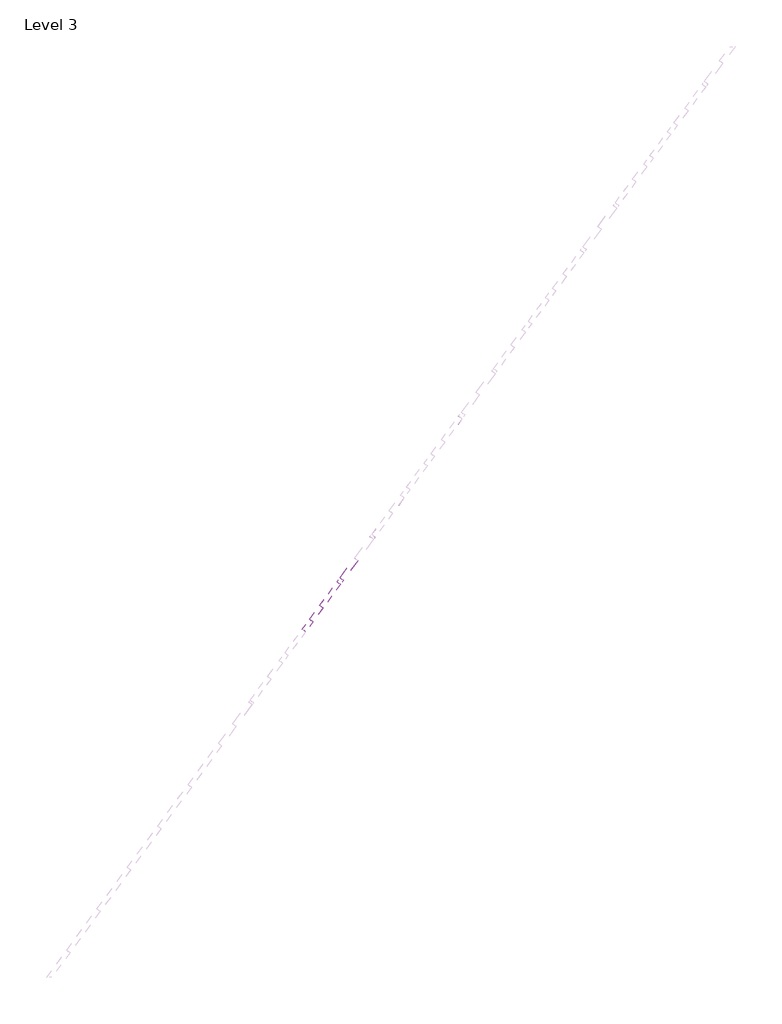
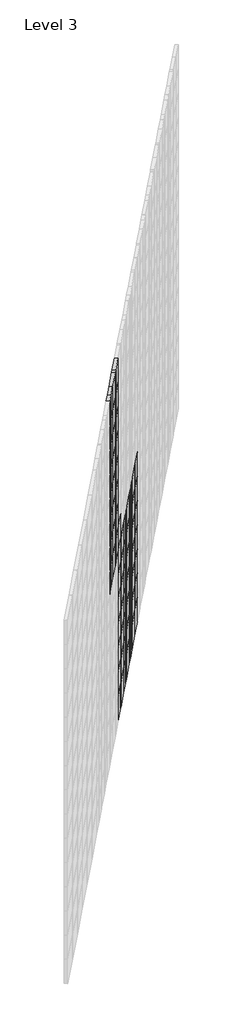
# One storey, part 5 of 9: 119 plates.
"""IFC4 building model written with IfcOpenShell, lengths in millimetres."""

import ifcopenshell
import ifcopenshell.guid

model = None  # the IFC model being written
_history = None  # IfcOwnerHistory: only IFC2X3 demands one
_inside = {}  # id of a spatial element -> (the spatial element, [elements in it])
_under = {}  # id of a project, library or spatial element -> (it, [spatial elements below it])
_declared = {}  # id of a project -> (the project, [libraries it declares])
_typed = {}  # id of a type object -> (the type object, [elements of that type])
_made_of = {}  # id of a material, layer set ... -> (it, [elements and type objects made of it])


def new_model(schema):
    """Start an empty IFC model of exactly this schema.

    Asked for "IFC4X3", IfcOpenShell would pick the latest addendum, in which some entities
    have other attributes; the version numbers below select the first issue.
    IFC2X3 requires an IfcOwnerHistory on every rooted entity: one is made here for all.
    """
    global model, _history
    if schema == "IFC4X3":
        model = ifcopenshell.file(schema_version=(4, 3, 0, 0))
    else:
        model = ifcopenshell.file(schema=schema)
    _inside.clear()
    _under.clear()
    _declared.clear()
    _typed.clear()
    _made_of.clear()
    _history = None
    if model.schema == "IFC2X3":
        org = make("IfcOrganization", Name="unknown")
        user = make(
            "IfcPersonAndOrganization",
            ThePerson=make("IfcPerson", FamilyName="unknown"),
            TheOrganization=org,
        )
        app = make(
            "IfcApplication",
            ApplicationDeveloper=org,
            Version="unknown",
            ApplicationFullName="unknown",
            ApplicationIdentifier="unknown",
        )
        _history = make(
            "IfcOwnerHistory",
            OwningUser=user,
            OwningApplication=app,
            ChangeAction="ADDED",
            CreationDate=0,
        )
    return model


def make(cls, **values):
    """One entity of the class cls with the attributes given. An attribute that is None is left unset."""
    return model.create_entity(
        cls, **{name: value for name, value in values.items() if value is not None}
    )


def rooted(cls, **values):
    """An entity with a GlobalId (a new one), such as an element, a storey or a relation."""
    return make(cls, GlobalId=ifcopenshell.guid.new(), OwnerHistory=_history, **values)


def si_unit(unit_type, name, prefix=None):
    """IfcSIUnit, for example si_unit("LENGTHUNIT", "METRE", prefix="MILLI")."""
    return make("IfcSIUnit", UnitType=unit_type, Prefix=prefix, Name=name)


def assignment(units):
    """IfcUnitAssignment: the units of a project."""
    return None if units is None else make("IfcUnitAssignment", Units=units)


def point(xyz):
    """IfcCartesianPoint."""
    return None if xyz is None else make("IfcCartesianPoint", Coordinates=xyz)


def direction(xyz):
    """IfcDirection."""
    return None if xyz is None else make("IfcDirection", DirectionRatios=xyz)


def frame(location, z_axis=None, x_axis=None):
    """IfcAxis2Placement3D, a coordinate frame: its origin and axes. An axis left out is left unset."""
    return make(
        "IfcAxis2Placement3D",
        Location=point(location),
        Axis=direction(z_axis),
        RefDirection=direction(x_axis),
    )


def origin():
    """The frame at (0, 0, 0) with its axes left unset."""
    return frame((0.0, 0.0, 0.0))


def origin_with_axes():
    """The frame at (0, 0, 0) with the z axis (0, 0, 1) and the x axis (1, 0, 0) written out."""
    return frame((0.0, 0.0, 0.0), z_axis=(0.0, 0.0, 1.0), x_axis=(1.0, 0.0, 0.0))


def place(relative_to, where):
    """IfcLocalPlacement: puts the frame where relative to a parent placement (None: the world)."""
    return make(
        "IfcLocalPlacement", PlacementRelTo=relative_to, RelativePlacement=where
    )


def context(
    kind, dimensions, precision=None, world=None, true_north=None, identifier=None
):
    """IfcGeometricRepresentationContext, for example the 3D "Model" context."""
    return make(
        "IfcGeometricRepresentationContext",
        ContextIdentifier=identifier,
        ContextType=kind,
        CoordinateSpaceDimension=dimensions,
        Precision=precision,
        WorldCoordinateSystem=world,
        TrueNorth=true_north,
    )


def project(units=None, contexts=None):
    """IfcProject with its units and contexts."""
    return rooted(
        "IfcProject",
        Name="project",
        RepresentationContexts=contexts,
        UnitsInContext=assignment(units),
    )


def spatial(cls, under=None, at=None, **own):
    """A site, building, storey or space (cls), placed at a placement, below another one or the project."""
    s = rooted(cls, ObjectPlacement=at, **own)
    if under is not None:
        _under.setdefault(under.id(), (under, []))[1].append(s)
    return s


def polyline(points):
    """IfcPolyline through the points."""
    return make("IfcPolyline", Points=[point(p) for p in points])


def outline(outer, holes=None, kind="AREA"):
    """IfcArbitraryClosedProfileDef: a profile drawn as a closed curve; with holes, ...WithVoids."""
    if holes is None:
        return make("IfcArbitraryClosedProfileDef", ProfileType=kind, OuterCurve=outer)
    return make(
        "IfcArbitraryProfileDefWithVoids",
        ProfileType=kind,
        OuterCurve=outer,
        InnerCurves=holes,
    )


def extrude(swept, where, along, depth):
    """IfcExtrudedAreaSolid: the profile swept, set in the frame where, extruded along a direction by depth."""
    return make(
        "IfcExtrudedAreaSolid",
        SweptArea=swept,
        Position=where,
        ExtrudedDirection=direction(along),
        Depth=depth,
    )


def shape(context_of_items, identifier, shape_type, items):
    """IfcShapeRepresentation: the items that make up one representation, for example the "Body"."""
    return make(
        "IfcShapeRepresentation",
        ContextOfItems=context_of_items,
        RepresentationIdentifier=identifier,
        RepresentationType=shape_type,
        Items=items,
    )


def source(mapping_origin, context_of_items, identifier, shape_type, items):
    """IfcRepresentationMap: a shape defined once, which mapped items show again and again."""
    return make(
        "IfcRepresentationMap",
        MappingOrigin=mapping_origin,
        MappedRepresentation=shape(context_of_items, identifier, shape_type, items),
    )


def transform(
    local_origin,
    x_axis=None,
    y_axis=None,
    z_axis=None,
    scale=None,
    scale2=None,
    scale3=None,
    uniform=True,
):
    """IfcCartesianTransformationOperator3D, or its non-uniform kind. x_axis, y_axis, z_axis: its Axis1, 2, 3."""
    if uniform:
        return make(
            "IfcCartesianTransformationOperator3D",
            Axis1=direction(x_axis),
            Axis2=direction(y_axis),
            LocalOrigin=point(local_origin),
            Scale=scale,
            Axis3=direction(z_axis),
        )
    return make(
        "IfcCartesianTransformationOperator3DnonUniform",
        Axis1=direction(x_axis),
        Axis2=direction(y_axis),
        LocalOrigin=point(local_origin),
        Scale=scale,
        Axis3=direction(z_axis),
        Scale2=scale2,
        Scale3=scale3,
    )


def mapped(mapping_source, mapping_target):
    """IfcMappedItem: shows the shape of a source again, moved by a transform."""
    return make(
        "IfcMappedItem", MappingSource=mapping_source, MappingTarget=mapping_target
    )


def made_of(thing, what):
    """Note that an element or type object is made of a material, layer set ...; save() writes the relation."""
    if what is not None:
        _made_of.setdefault(what.id(), (what, []))[1].append(thing)
    return thing


def element(
    cls,
    number,
    at=None,
    inside=None,
    cuts=None,
    type_object=None,
    material=None,
    context=None,
    identifier="Body",
    shape_type=None,
    held_by="IfcProductDefinitionShape",
    body=None,
    shapes=None,
    **own,
):
    """One element of the class cls, such as IfcWall. Its Tag is "e" and its number.

    at: its placement. inside: the storey or other place that contains it. cuts: it is an
    opening in that element (IfcRelVoidsElement). A single representation is given by context,
    identifier, shape_type and body (its items); several are given by shapes. held_by: the class
    of the entity that holds the representations. save() writes the other relations.
    """
    e = rooted(cls, Tag="e%d" % number, ObjectPlacement=at, **own)
    if body is not None:
        shapes = [shape(context, identifier, shape_type, body)]
    if shapes is not None:
        e.Representation = make(held_by, Representations=shapes)
    if inside is not None:
        _inside.setdefault(inside.id(), (inside, []))[1].append(e)
    if cuts is not None:
        rooted(
            "IfcRelVoidsElement", RelatingBuildingElement=cuts, RelatedOpeningElement=e
        )
    if type_object is not None:
        _typed.setdefault(type_object.id(), (type_object, []))[1].append(e)
    return made_of(e, material)


def aggregate(whole, parts):
    """IfcRelAggregates: a whole, such as a stair, and the parts it consists of."""
    return rooted("IfcRelAggregates", RelatingObject=whole, RelatedObjects=parts)


def save(model, path):
    """Write the relations noted so far, then the file.

    IfcRelAggregates (storeys below a building ...), IfcRelContainedInSpatialStructure (elements
    in a storey), IfcRelDefinesByType, IfcRelAssociatesMaterial and IfcRelDeclares: one each for
    every whole, place, type object, material and project.
    """
    for whole, parts in _under.values():
        aggregate(whole, parts)
    for where, things in _inside.values():
        rooted(
            "IfcRelContainedInSpatialStructure",
            RelatedElements=things,
            RelatingStructure=where,
        )
    for kind, things in _typed.values():
        rooted("IfcRelDefinesByType", RelatedObjects=things, RelatingType=kind)
    for what, things in _made_of.values():
        rooted("IfcRelAssociatesMaterial", RelatedObjects=things, RelatingMaterial=what)
    for by, libraries in _declared.values():
        rooted("IfcRelDeclares", RelatingContext=by, RelatedDefinitions=libraries)
    model.write(path)


def system_panel_glazed_3dd544b4(model_context):
    return source(origin(), model_context, "Body", "SweptSolid", [
        extrude(outline(polyline([(49.4357818, 24.5), (-49.4357818, 24.5), (-49.4357818, 49.5), (49.4357818, 49.5), (49.4357818, 24.5)])), origin_with_axes(), (0.0, 0.0, 1.0), 200.0),
    ])


def system_panel_glazed_de50ea70(model_context):
    return source(origin(), model_context, "Body", "SweptSolid", [
        extrude(outline(polyline([(70.9525426, 24.5), (-70.9525426, 24.5), (-70.9525426, 49.5), (70.9525426, 49.5), (70.9525426, 24.5)])), origin_with_axes(), (0.0, 0.0, 1.0), 200.0),
    ])


def system_panel_glazed_3bc540b8(model_context):
    return source(origin(), model_context, "Body", "SweptSolid", [
        extrude(outline(polyline([(7.4693035, 24.5), (-7.4693035, 24.5), (-7.4693035, 49.5), (7.4693035, 49.5), (7.4693035, 24.5)])), origin_with_axes(), (0.0, 0.0, 1.0), 200.0),
    ])


def system_panel_glazed_0948c99b(model_context):
    return source(origin(), model_context, "Body", "SweptSolid", [
        extrude(outline(polyline([(28.9860643, 24.5), (-28.9860643, 24.5), (-28.9860643, 49.5), (28.9860643, 49.5), (28.9860643, 24.5)])), origin_with_axes(), (0.0, 0.0, 1.0), 200.0),
    ])


def system_panel_glazed_b9ee7cbb(model_context):
    return source(origin(), model_context, "Body", "SweptSolid", [
        extrude(outline(polyline([(50.5028251, 24.5), (-50.5028251, 24.5), (-50.5028251, 49.5), (50.5028251, 49.5), (50.5028251, 24.5)])), origin_with_axes(), (0.0, 0.0, 1.0), 200.0),
    ])


def system_panel_glazed_192fb397(model_context):
    return source(origin(), model_context, "Body", "SweptSolid", [
        extrude(outline(polyline([(72.019586, 24.5), (-72.019586, 24.5), (-72.019586, 49.5), (72.019586, 49.5), (72.019586, 24.5)])), origin_with_axes(), (0.0, 0.0, 1.0), 200.0),
    ])


def system_panel_glazed_1ea8d406(model_context):
    return source(origin(), model_context, "Body", "SweptSolid", [
        extrude(outline(polyline([(85.0, 24.5), (-85.0, 24.5), (-85.0, 49.5), (85.0, 49.5), (85.0, 24.5)])), origin_with_axes(), (0.0, 0.0, 1.0), 200.0),
    ])


def system_panel_glazed_d81ce811(model_context):
    return source(origin(), model_context, "Body", "SweptSolid", [
        extrude(outline(polyline([(35.5642182, 24.5), (-35.5642182, 24.5), (-35.5642182, 49.5), (35.5642182, 49.5), (35.5642182, 24.5)])), origin_with_axes(), (0.0, 0.0, 1.0), 200.0),
    ])


def system_panel_glazed_acae83c8(model_context):
    return source(origin(), model_context, "Body", "SweptSolid", [
        extrude(outline(polyline([(14.0474574, 24.5), (-14.0474574, 24.5), (-14.0474574, 49.5), (14.0474574, 49.5), (14.0474574, 24.5)])), origin_with_axes(), (0.0, 0.0, 1.0), 200.0),
    ])


def system_panel_glazed_83ffeb2f(model_context):
    return source(origin(), model_context, "Body", "SweptSolid", [
        extrude(outline(polyline([(77.5306965, 24.5), (-77.5306965, 24.5), (-77.5306965, 49.5), (77.5306965, 49.5), (77.5306965, 24.5)])), origin_with_axes(), (0.0, 0.0, 1.0), 200.0),
    ])


def system_panel_glazed_1aaa8be2(model_context):
    return source(origin(), model_context, "Body", "SweptSolid", [
        extrude(outline(polyline([(56.0139357, 24.5), (-56.0139357, 24.5), (-56.0139357, 49.5), (56.0139357, 49.5), (56.0139357, 24.5)])), origin_with_axes(), (0.0, 0.0, 1.0), 200.0),
    ])


def system_panel_glazed_efe9a4c3(model_context):
    return source(origin(), model_context, "Body", "SweptSolid", [
        extrude(outline(polyline([(34.4971749, 24.5), (-34.4971749, 24.5), (-34.4971749, 49.5), (34.4971749, 49.5), (34.4971749, 24.5)])), origin_with_axes(), (0.0, 0.0, 1.0), 200.0),
    ])


def system_panel_glazed_b8c9dfa1(model_context):
    return source(origin(), model_context, "Body", "SweptSolid", [
        extrude(outline(polyline([(12.980414, 24.5), (-12.980414, 24.5), (-12.980414, 49.5), (12.980414, 49.5), (12.980414, 24.5)])), origin_with_axes(), (0.0, 0.0, 1.0), 200.0),
    ])


model = new_model("IFC4")

# Units and contexts
model_context = context("Model", 3, world=origin())
ifc_project = project(units=[si_unit("LENGTHUNIT", "METRE", prefix="MILLI")], contexts=[model_context])

# Site, building, storey
site = spatial("IfcSite", under=ifc_project)
building = spatial("IfcBuilding", under=site)
storey = spatial("IfcBuildingStorey", under=building, Name="Level 3", Elevation=22950.0)

# Plates
placement = place(None, origin())
system_panel_glazed_shape = system_panel_glazed_3dd544b4(model_context)
element("IfcPlate", 1, ObjectType="System Panel : Glazed", at=placement, inside=storey, context=model_context, shape_type="MappedRepresentation", body=[
    mapped(system_panel_glazed_shape, transform((-32903.673453, 28665.1875834, 36500.0), x_axis=(0.5920548138930122, 0.8058976965757569, 0.0), y_axis=(-0.8058976965757569, 0.5920548138930122, 0.0), z_axis=(0.0, 0.0, 1.0))),
])
element("IfcPlate", 2, ObjectType="System Panel : Glazed", at=placement, inside=storey, context=model_context, shape_type="MappedRepresentation", body=[
    mapped(system_panel_glazed_shape, transform((-32903.673453, 28665.1875834, 36700.0), x_axis=(0.5920548138930122, 0.8058976965757569, 0.0), y_axis=(-0.8058976965757569, 0.5920548138930122, 0.0), z_axis=(0.0, 0.0, 1.0))),
])
element("IfcPlate", 3, ObjectType="System Panel : Glazed", at=placement, inside=storey, context=model_context, shape_type="MappedRepresentation", body=[
    mapped(system_panel_glazed_shape, transform((-32903.673453, 28665.1875834, 36900.0), x_axis=(0.5920548138930122, 0.8058976965757569, 0.0), y_axis=(-0.8058976965757569, 0.5920548138930122, 0.0), z_axis=(0.0, 0.0, 1.0))),
])
element("IfcPlate", 4, ObjectType="System Panel : Glazed", at=placement, inside=storey, context=model_context, shape_type="MappedRepresentation", body=[
    mapped(system_panel_glazed_shape, transform((-32903.673453, 28665.1875834, 37100.0), x_axis=(0.5920548138930122, 0.8058976965757569, 0.0), y_axis=(-0.8058976965757569, 0.5920548138930122, 0.0), z_axis=(0.0, 0.0, 1.0))),
])
element("IfcPlate", 5, ObjectType="System Panel : Glazed", at=placement, inside=storey, context=model_context, shape_type="MappedRepresentation", body=[
    mapped(system_panel_glazed_shape, transform((-32903.673453, 28665.1875834, 37300.0), x_axis=(0.5920548138930122, 0.8058976965757569, 0.0), y_axis=(-0.8058976965757569, 0.5920548138930122, 0.0), z_axis=(0.0, 0.0, 1.0))),
])
element("IfcPlate", 6, ObjectType="System Panel : Glazed", at=placement, inside=storey, context=model_context, shape_type="MappedRepresentation", body=[
    mapped(system_panel_glazed_shape, transform((-32903.673453, 28665.1875834, 37500.0), x_axis=(0.5920548138930122, 0.8058976965757569, 0.0), y_axis=(-0.8058976965757569, 0.5920548138930122, 0.0), z_axis=(0.0, 0.0, 1.0))),
])
element("IfcPlate", 7, ObjectType="System Panel : Glazed", at=placement, inside=storey, context=model_context, shape_type="MappedRepresentation", body=[
    mapped(system_panel_glazed_shape, transform((-32903.673453, 28665.1875834, 37700.0), x_axis=(0.5920548138930122, 0.8058976965757569, 0.0), y_axis=(-0.8058976965757569, 0.5920548138930122, 0.0), z_axis=(0.0, 0.0, 1.0))),
])
element("IfcPlate", 8, ObjectType="System Panel : Glazed", at=placement, inside=storey, context=model_context, shape_type="MappedRepresentation", body=[
    mapped(system_panel_glazed_shape, transform((-32903.673453, 28665.1875834, 37900.0), x_axis=(0.5920548138930122, 0.8058976965757569, 0.0), y_axis=(-0.8058976965757569, 0.5920548138930122, 0.0), z_axis=(0.0, 0.0, 1.0))),
])
system_panel_glazed_2_shape = system_panel_glazed_de50ea70(model_context)
element("IfcPlate", 9, ObjectType="System Panel : Glazed", at=placement, inside=storey, context=model_context, shape_type="MappedRepresentation", body=[
    mapped(system_panel_glazed_2_shape, transform((-32715.1139181, 28921.8524922, 36500.0), x_axis=(0.5920548138930122, 0.8058976965757569, 0.0), y_axis=(-0.8058976965757569, 0.5920548138930122, 0.0), z_axis=(0.0, 0.0, 1.0))),
])
element("IfcPlate", 10, ObjectType="System Panel : Glazed", at=placement, inside=storey, context=model_context, shape_type="MappedRepresentation", body=[
    mapped(system_panel_glazed_2_shape, transform((-32715.1139181, 28921.8524922, 36700.0), x_axis=(0.5920548138930122, 0.8058976965757569, 0.0), y_axis=(-0.8058976965757569, 0.5920548138930122, 0.0), z_axis=(0.0, 0.0, 1.0))),
])
element("IfcPlate", 11, ObjectType="System Panel : Glazed", at=placement, inside=storey, context=model_context, shape_type="MappedRepresentation", body=[
    mapped(system_panel_glazed_2_shape, transform((-32715.1139181, 28921.8524922, 36900.0), x_axis=(0.5920548138930122, 0.8058976965757569, 0.0), y_axis=(-0.8058976965757569, 0.5920548138930122, 0.0), z_axis=(0.0, 0.0, 1.0))),
])
element("IfcPlate", 12, ObjectType="System Panel : Glazed", at=placement, inside=storey, context=model_context, shape_type="MappedRepresentation", body=[
    mapped(system_panel_glazed_2_shape, transform((-32715.1139181, 28921.8524922, 37100.0), x_axis=(0.5920548138930122, 0.8058976965757569, 0.0), y_axis=(-0.8058976965757569, 0.5920548138930122, 0.0), z_axis=(0.0, 0.0, 1.0))),
])
element("IfcPlate", 13, ObjectType="System Panel : Glazed", at=placement, inside=storey, context=model_context, shape_type="MappedRepresentation", body=[
    mapped(system_panel_glazed_2_shape, transform((-32715.1139181, 28921.8524922, 37300.0), x_axis=(0.5920548138930122, 0.8058976965757569, 0.0), y_axis=(-0.8058976965757569, 0.5920548138930122, 0.0), z_axis=(0.0, 0.0, 1.0))),
])
element("IfcPlate", 14, ObjectType="System Panel : Glazed", at=placement, inside=storey, context=model_context, shape_type="MappedRepresentation", body=[
    mapped(system_panel_glazed_2_shape, transform((-32715.1139181, 28921.8524922, 37500.0), x_axis=(0.5920548138930122, 0.8058976965757569, 0.0), y_axis=(-0.8058976965757569, 0.5920548138930122, 0.0), z_axis=(0.0, 0.0, 1.0))),
])
element("IfcPlate", 15, ObjectType="System Panel : Glazed", at=placement, inside=storey, context=model_context, shape_type="MappedRepresentation", body=[
    mapped(system_panel_glazed_2_shape, transform((-32715.1139181, 28921.8524922, 37700.0), x_axis=(0.5920548138930122, 0.8058976965757569, 0.0), y_axis=(-0.8058976965757569, 0.5920548138930122, 0.0), z_axis=(0.0, 0.0, 1.0))),
])
element("IfcPlate", 16, ObjectType="System Panel : Glazed", at=placement, inside=storey, context=model_context, shape_type="MappedRepresentation", body=[
    mapped(system_panel_glazed_2_shape, transform((-32715.1139181, 28921.8524922, 37900.0), x_axis=(0.5920548138930122, 0.8058976965757569, 0.0), y_axis=(-0.8058976965757569, 0.5920548138930122, 0.0), z_axis=(0.0, 0.0, 1.0))),
])
system_panel_glazed_3_shape = system_panel_glazed_3bc540b8(model_context)
element("IfcPlate", 17, ObjectType="System Panel : Glazed", at=placement, inside=storey, context=model_context, shape_type="MappedRepresentation", body=[
    mapped(system_panel_glazed_3_shape, transform((-32576.8790424, 29110.0160968, 35100.0), x_axis=(0.5920548138930122, 0.8058976965757569, 0.0), y_axis=(-0.8058976965757569, 0.5920548138930122, 0.0), z_axis=(0.0, 0.0, 1.0))),
])
element("IfcPlate", 18, ObjectType="System Panel : Glazed", at=placement, inside=storey, context=model_context, shape_type="MappedRepresentation", body=[
    mapped(system_panel_glazed_3_shape, transform((-32576.8790424, 29110.0160968, 35300.0), x_axis=(0.5920548138930122, 0.8058976965757569, 0.0), y_axis=(-0.8058976965757569, 0.5920548138930122, 0.0), z_axis=(0.0, 0.0, 1.0))),
])
element("IfcPlate", 19, ObjectType="System Panel : Glazed", at=placement, inside=storey, context=model_context, shape_type="MappedRepresentation", body=[
    mapped(system_panel_glazed_3_shape, transform((-32576.8790424, 29110.0160968, 35500.0), x_axis=(0.5920548138930122, 0.8058976965757569, 0.0), y_axis=(-0.8058976965757569, 0.5920548138930122, 0.0), z_axis=(0.0, 0.0, 1.0))),
])
element("IfcPlate", 20, ObjectType="System Panel : Glazed", at=placement, inside=storey, context=model_context, shape_type="MappedRepresentation", body=[
    mapped(system_panel_glazed_3_shape, transform((-32576.8790424, 29110.0160968, 35700.0), x_axis=(0.5920548138930122, 0.8058976965757569, 0.0), y_axis=(-0.8058976965757569, 0.5920548138930122, 0.0), z_axis=(0.0, 0.0, 1.0))),
])
element("IfcPlate", 21, ObjectType="System Panel : Glazed", at=placement, inside=storey, context=model_context, shape_type="MappedRepresentation", body=[
    mapped(system_panel_glazed_3_shape, transform((-32576.8790424, 29110.0160968, 35900.0), x_axis=(0.5920548138930122, 0.8058976965757569, 0.0), y_axis=(-0.8058976965757569, 0.5920548138930122, 0.0), z_axis=(0.0, 0.0, 1.0))),
])
element("IfcPlate", 22, ObjectType="System Panel : Glazed", at=placement, inside=storey, context=model_context, shape_type="MappedRepresentation", body=[
    mapped(system_panel_glazed_3_shape, transform((-32576.8790424, 29110.0160968, 36100.0), x_axis=(0.5920548138930122, 0.8058976965757569, 0.0), y_axis=(-0.8058976965757569, 0.5920548138930122, 0.0), z_axis=(0.0, 0.0, 1.0))),
])
element("IfcPlate", 23, ObjectType="System Panel : Glazed", at=placement, inside=storey, context=model_context, shape_type="MappedRepresentation", body=[
    mapped(system_panel_glazed_3_shape, transform((-32576.8790424, 29110.0160968, 36300.0), x_axis=(0.5920548138930122, 0.8058976965757569, 0.0), y_axis=(-0.8058976965757569, 0.5920548138930122, 0.0), z_axis=(0.0, 0.0, 1.0))),
])
element("IfcPlate", 24, ObjectType="System Panel : Glazed", at=placement, inside=storey, context=model_context, shape_type="MappedRepresentation", body=[
    mapped(system_panel_glazed_3_shape, transform((-32576.8790424, 29110.0160968, 36500.0), x_axis=(0.5920548138930122, 0.8058976965757569, 0.0), y_axis=(-0.8058976965757569, 0.5920548138930122, 0.0), z_axis=(0.0, 0.0, 1.0))),
])
system_panel_glazed_4_shape = system_panel_glazed_0948c99b(model_context)
element("IfcPlate", 25, ObjectType="System Panel : Glazed", at=placement, inside=storey, context=model_context, shape_type="MappedRepresentation", body=[
    mapped(system_panel_glazed_4_shape, transform((-32388.3195075, 29366.6810057, 35100.0), x_axis=(0.5920548138930122, 0.8058976965757569, 0.0), y_axis=(-0.8058976965757569, 0.5920548138930122, 0.0), z_axis=(0.0, 0.0, 1.0))),
])
element("IfcPlate", 26, ObjectType="System Panel : Glazed", at=placement, inside=storey, context=model_context, shape_type="MappedRepresentation", body=[
    mapped(system_panel_glazed_4_shape, transform((-32388.3195075, 29366.6810057, 35300.0), x_axis=(0.5920548138930122, 0.8058976965757569, 0.0), y_axis=(-0.8058976965757569, 0.5920548138930122, 0.0), z_axis=(0.0, 0.0, 1.0))),
])
element("IfcPlate", 27, ObjectType="System Panel : Glazed", at=placement, inside=storey, context=model_context, shape_type="MappedRepresentation", body=[
    mapped(system_panel_glazed_4_shape, transform((-32388.3195075, 29366.6810057, 35500.0), x_axis=(0.5920548138930122, 0.8058976965757569, 0.0), y_axis=(-0.8058976965757569, 0.5920548138930122, 0.0), z_axis=(0.0, 0.0, 1.0))),
])
element("IfcPlate", 28, ObjectType="System Panel : Glazed", at=placement, inside=storey, context=model_context, shape_type="MappedRepresentation", body=[
    mapped(system_panel_glazed_4_shape, transform((-32388.3195075, 29366.6810057, 35700.0), x_axis=(0.5920548138930122, 0.8058976965757569, 0.0), y_axis=(-0.8058976965757569, 0.5920548138930122, 0.0), z_axis=(0.0, 0.0, 1.0))),
])
element("IfcPlate", 29, ObjectType="System Panel : Glazed", at=placement, inside=storey, context=model_context, shape_type="MappedRepresentation", body=[
    mapped(system_panel_glazed_4_shape, transform((-32388.3195075, 29366.6810057, 35900.0), x_axis=(0.5920548138930122, 0.8058976965757569, 0.0), y_axis=(-0.8058976965757569, 0.5920548138930122, 0.0), z_axis=(0.0, 0.0, 1.0))),
])
element("IfcPlate", 30, ObjectType="System Panel : Glazed", at=placement, inside=storey, context=model_context, shape_type="MappedRepresentation", body=[
    mapped(system_panel_glazed_4_shape, transform((-32388.3195075, 29366.6810057, 36100.0), x_axis=(0.5920548138930122, 0.8058976965757569, 0.0), y_axis=(-0.8058976965757569, 0.5920548138930122, 0.0), z_axis=(0.0, 0.0, 1.0))),
])
element("IfcPlate", 31, ObjectType="System Panel : Glazed", at=placement, inside=storey, context=model_context, shape_type="MappedRepresentation", body=[
    mapped(system_panel_glazed_4_shape, transform((-32388.3195075, 29366.6810057, 36300.0), x_axis=(0.5920548138930122, 0.8058976965757569, 0.0), y_axis=(-0.8058976965757569, 0.5920548138930122, 0.0), z_axis=(0.0, 0.0, 1.0))),
])
system_panel_glazed_5_shape = system_panel_glazed_b9ee7cbb(model_context)
element("IfcPlate", 32, ObjectType="System Panel : Glazed", at=placement, inside=storey, context=model_context, shape_type="MappedRepresentation", body=[
    mapped(system_panel_glazed_5_shape, transform((-32199.7599726, 29623.3459145, 35100.0), x_axis=(0.5920548138930122, 0.8058976965757569, 0.0), y_axis=(-0.8058976965757569, 0.5920548138930122, 0.0), z_axis=(0.0, 0.0, 1.0))),
])
element("IfcPlate", 33, ObjectType="System Panel : Glazed", at=placement, inside=storey, context=model_context, shape_type="MappedRepresentation", body=[
    mapped(system_panel_glazed_5_shape, transform((-32199.7599726, 29623.3459145, 35300.0), x_axis=(0.5920548138930122, 0.8058976965757569, 0.0), y_axis=(-0.8058976965757569, 0.5920548138930122, 0.0), z_axis=(0.0, 0.0, 1.0))),
])
element("IfcPlate", 34, ObjectType="System Panel : Glazed", at=placement, inside=storey, context=model_context, shape_type="MappedRepresentation", body=[
    mapped(system_panel_glazed_5_shape, transform((-32199.7599726, 29623.3459145, 35500.0), x_axis=(0.5920548138930122, 0.8058976965757569, 0.0), y_axis=(-0.8058976965757569, 0.5920548138930122, 0.0), z_axis=(0.0, 0.0, 1.0))),
])
element("IfcPlate", 35, ObjectType="System Panel : Glazed", at=placement, inside=storey, context=model_context, shape_type="MappedRepresentation", body=[
    mapped(system_panel_glazed_5_shape, transform((-32199.7599726, 29623.3459145, 35700.0), x_axis=(0.5920548138930122, 0.8058976965757569, 0.0), y_axis=(-0.8058976965757569, 0.5920548138930122, 0.0), z_axis=(0.0, 0.0, 1.0))),
])
element("IfcPlate", 36, ObjectType="System Panel : Glazed", at=placement, inside=storey, context=model_context, shape_type="MappedRepresentation", body=[
    mapped(system_panel_glazed_5_shape, transform((-32199.7599726, 29623.3459145, 35900.0), x_axis=(0.5920548138930122, 0.8058976965757569, 0.0), y_axis=(-0.8058976965757569, 0.5920548138930122, 0.0), z_axis=(0.0, 0.0, 1.0))),
])
element("IfcPlate", 37, ObjectType="System Panel : Glazed", at=placement, inside=storey, context=model_context, shape_type="MappedRepresentation", body=[
    mapped(system_panel_glazed_5_shape, transform((-32199.7599726, 29623.3459145, 36100.0), x_axis=(0.5920548138930122, 0.8058976965757569, 0.0), y_axis=(-0.8058976965757569, 0.5920548138930122, 0.0), z_axis=(0.0, 0.0, 1.0))),
])
element("IfcPlate", 38, ObjectType="System Panel : Glazed", at=placement, inside=storey, context=model_context, shape_type="MappedRepresentation", body=[
    mapped(system_panel_glazed_5_shape, transform((-32199.7599726, 29623.3459145, 36300.0), x_axis=(0.5920548138930122, 0.8058976965757569, 0.0), y_axis=(-0.8058976965757569, 0.5920548138930122, 0.0), z_axis=(0.0, 0.0, 1.0))),
])
system_panel_glazed_6_shape = system_panel_glazed_192fb397(model_context)
element("IfcPlate", 39, ObjectType="System Panel : Glazed", at=placement, inside=storey, context=model_context, shape_type="MappedRepresentation", body=[
    mapped(system_panel_glazed_6_shape, transform((-32011.2004377, 29880.0108233, 35100.0), x_axis=(0.5920548138930122, 0.8058976965757569, 0.0), y_axis=(-0.8058976965757569, 0.5920548138930122, 0.0), z_axis=(0.0, 0.0, 1.0))),
])
element("IfcPlate", 40, ObjectType="System Panel : Glazed", at=placement, inside=storey, context=model_context, shape_type="MappedRepresentation", body=[
    mapped(system_panel_glazed_6_shape, transform((-32011.2004377, 29880.0108233, 35300.0), x_axis=(0.5920548138930122, 0.8058976965757569, 0.0), y_axis=(-0.8058976965757569, 0.5920548138930122, 0.0), z_axis=(0.0, 0.0, 1.0))),
])
element("IfcPlate", 41, ObjectType="System Panel : Glazed", at=placement, inside=storey, context=model_context, shape_type="MappedRepresentation", body=[
    mapped(system_panel_glazed_6_shape, transform((-32011.2004377, 29880.0108233, 35500.0), x_axis=(0.5920548138930122, 0.8058976965757569, 0.0), y_axis=(-0.8058976965757569, 0.5920548138930122, 0.0), z_axis=(0.0, 0.0, 1.0))),
])
element("IfcPlate", 42, ObjectType="System Panel : Glazed", at=placement, inside=storey, context=model_context, shape_type="MappedRepresentation", body=[
    mapped(system_panel_glazed_6_shape, transform((-32011.2004377, 29880.0108233, 35700.0), x_axis=(0.5920548138930122, 0.8058976965757569, 0.0), y_axis=(-0.8058976965757569, 0.5920548138930122, 0.0), z_axis=(0.0, 0.0, 1.0))),
])
element("IfcPlate", 43, ObjectType="System Panel : Glazed", at=placement, inside=storey, context=model_context, shape_type="MappedRepresentation", body=[
    mapped(system_panel_glazed_6_shape, transform((-32011.2004377, 29880.0108233, 35900.0), x_axis=(0.5920548138930122, 0.8058976965757569, 0.0), y_axis=(-0.8058976965757569, 0.5920548138930122, 0.0), z_axis=(0.0, 0.0, 1.0))),
])
element("IfcPlate", 44, ObjectType="System Panel : Glazed", at=placement, inside=storey, context=model_context, shape_type="MappedRepresentation", body=[
    mapped(system_panel_glazed_6_shape, transform((-32011.2004377, 29880.0108233, 36100.0), x_axis=(0.5920548138930122, 0.8058976965757569, 0.0), y_axis=(-0.8058976965757569, 0.5920548138930122, 0.0), z_axis=(0.0, 0.0, 1.0))),
])
element("IfcPlate", 45, ObjectType="System Panel : Glazed", at=placement, inside=storey, context=model_context, shape_type="MappedRepresentation", body=[
    mapped(system_panel_glazed_6_shape, transform((-32011.2004377, 29880.0108233, 36300.0), x_axis=(0.5920548138930122, 0.8058976965757569, 0.0), y_axis=(-0.8058976965757569, 0.5920548138930122, 0.0), z_axis=(0.0, 0.0, 1.0))),
])
system_panel_glazed_7_shape = system_panel_glazed_1ea8d406(model_context)
element("IfcPlate", 46, ObjectType="System Panel : Glazed", at=placement, inside=storey, context=model_context, shape_type="MappedRepresentation", body=[
    mapped(system_panel_glazed_7_shape, transform((-32522.1321461, 29184.5368955, 35100.0), x_axis=(0.5920548138930122, 0.8058976965757569, 0.0), y_axis=(-0.8058976965757569, 0.5920548138930122, 0.0), z_axis=(0.0, 0.0, 1.0))),
])
element("IfcPlate", 47, ObjectType="System Panel : Glazed", at=placement, inside=storey, context=model_context, shape_type="MappedRepresentation", body=[
    mapped(system_panel_glazed_7_shape, transform((-32320.8335094, 29458.5421123, 35100.0), x_axis=(0.5920548138930122, 0.8058976965757569, 0.0), y_axis=(-0.8058976965757569, 0.5920548138930122, 0.0), z_axis=(0.0, 0.0, 1.0))),
])
element("IfcPlate", 48, ObjectType="System Panel : Glazed", at=placement, inside=storey, context=model_context, shape_type="MappedRepresentation", body=[
    mapped(system_panel_glazed_7_shape, transform((-32119.5348727, 29732.5473292, 35100.0), x_axis=(0.5920548138930122, 0.8058976965757569, 0.0), y_axis=(-0.8058976965757569, 0.5920548138930122, 0.0), z_axis=(0.0, 0.0, 1.0))),
])
element("IfcPlate", 49, ObjectType="System Panel : Glazed", at=placement, inside=storey, context=model_context, shape_type="MappedRepresentation", body=[
    mapped(system_panel_glazed_7_shape, transform((-32522.1321461, 29184.5368955, 35300.0), x_axis=(0.5920548138930122, 0.8058976965757569, 0.0), y_axis=(-0.8058976965757569, 0.5920548138930122, 0.0), z_axis=(0.0, 0.0, 1.0))),
])
element("IfcPlate", 50, ObjectType="System Panel : Glazed", at=placement, inside=storey, context=model_context, shape_type="MappedRepresentation", body=[
    mapped(system_panel_glazed_7_shape, transform((-32320.8335094, 29458.5421123, 35300.0), x_axis=(0.5920548138930122, 0.8058976965757569, 0.0), y_axis=(-0.8058976965757569, 0.5920548138930122, 0.0), z_axis=(0.0, 0.0, 1.0))),
])
element("IfcPlate", 51, ObjectType="System Panel : Glazed", at=placement, inside=storey, context=model_context, shape_type="MappedRepresentation", body=[
    mapped(system_panel_glazed_7_shape, transform((-32119.5348727, 29732.5473292, 35300.0), x_axis=(0.5920548138930122, 0.8058976965757569, 0.0), y_axis=(-0.8058976965757569, 0.5920548138930122, 0.0), z_axis=(0.0, 0.0, 1.0))),
])
element("IfcPlate", 52, ObjectType="System Panel : Glazed", at=placement, inside=storey, context=model_context, shape_type="MappedRepresentation", body=[
    mapped(system_panel_glazed_7_shape, transform((-32522.1321461, 29184.5368955, 35500.0), x_axis=(0.5920548138930122, 0.8058976965757569, 0.0), y_axis=(-0.8058976965757569, 0.5920548138930122, 0.0), z_axis=(0.0, 0.0, 1.0))),
])
element("IfcPlate", 53, ObjectType="System Panel : Glazed", at=placement, inside=storey, context=model_context, shape_type="MappedRepresentation", body=[
    mapped(system_panel_glazed_7_shape, transform((-32320.8335094, 29458.5421123, 35500.0), x_axis=(0.5920548138930122, 0.8058976965757569, 0.0), y_axis=(-0.8058976965757569, 0.5920548138930122, 0.0), z_axis=(0.0, 0.0, 1.0))),
])
element("IfcPlate", 54, ObjectType="System Panel : Glazed", at=placement, inside=storey, context=model_context, shape_type="MappedRepresentation", body=[
    mapped(system_panel_glazed_7_shape, transform((-32119.5348727, 29732.5473292, 35500.0), x_axis=(0.5920548138930122, 0.8058976965757569, 0.0), y_axis=(-0.8058976965757569, 0.5920548138930122, 0.0), z_axis=(0.0, 0.0, 1.0))),
])
element("IfcPlate", 55, ObjectType="System Panel : Glazed", at=placement, inside=storey, context=model_context, shape_type="MappedRepresentation", body=[
    mapped(system_panel_glazed_7_shape, transform((-32522.1321461, 29184.5368955, 35700.0), x_axis=(0.5920548138930122, 0.8058976965757569, 0.0), y_axis=(-0.8058976965757569, 0.5920548138930122, 0.0), z_axis=(0.0, 0.0, 1.0))),
])
element("IfcPlate", 56, ObjectType="System Panel : Glazed", at=placement, inside=storey, context=model_context, shape_type="MappedRepresentation", body=[
    mapped(system_panel_glazed_7_shape, transform((-32320.8335094, 29458.5421123, 35700.0), x_axis=(0.5920548138930122, 0.8058976965757569, 0.0), y_axis=(-0.8058976965757569, 0.5920548138930122, 0.0), z_axis=(0.0, 0.0, 1.0))),
])
element("IfcPlate", 57, ObjectType="System Panel : Glazed", at=placement, inside=storey, context=model_context, shape_type="MappedRepresentation", body=[
    mapped(system_panel_glazed_7_shape, transform((-32119.5348727, 29732.5473292, 35700.0), x_axis=(0.5920548138930122, 0.8058976965757569, 0.0), y_axis=(-0.8058976965757569, 0.5920548138930122, 0.0), z_axis=(0.0, 0.0, 1.0))),
])
element("IfcPlate", 58, ObjectType="System Panel : Glazed", at=placement, inside=storey, context=model_context, shape_type="MappedRepresentation", body=[
    mapped(system_panel_glazed_7_shape, transform((-32522.1321461, 29184.5368955, 35900.0), x_axis=(0.5920548138930122, 0.8058976965757569, 0.0), y_axis=(-0.8058976965757569, 0.5920548138930122, 0.0), z_axis=(0.0, 0.0, 1.0))),
])
element("IfcPlate", 59, ObjectType="System Panel : Glazed", at=placement, inside=storey, context=model_context, shape_type="MappedRepresentation", body=[
    mapped(system_panel_glazed_7_shape, transform((-32320.8335094, 29458.5421123, 35900.0), x_axis=(0.5920548138930122, 0.8058976965757569, 0.0), y_axis=(-0.8058976965757569, 0.5920548138930122, 0.0), z_axis=(0.0, 0.0, 1.0))),
])
element("IfcPlate", 60, ObjectType="System Panel : Glazed", at=placement, inside=storey, context=model_context, shape_type="MappedRepresentation", body=[
    mapped(system_panel_glazed_7_shape, transform((-32119.5348727, 29732.5473292, 35900.0), x_axis=(0.5920548138930122, 0.8058976965757569, 0.0), y_axis=(-0.8058976965757569, 0.5920548138930122, 0.0), z_axis=(0.0, 0.0, 1.0))),
])
element("IfcPlate", 61, ObjectType="System Panel : Glazed", at=placement, inside=storey, context=model_context, shape_type="MappedRepresentation", body=[
    mapped(system_panel_glazed_7_shape, transform((-32522.1321461, 29184.5368955, 36100.0), x_axis=(0.5920548138930122, 0.8058976965757569, 0.0), y_axis=(-0.8058976965757569, 0.5920548138930122, 0.0), z_axis=(0.0, 0.0, 1.0))),
])
element("IfcPlate", 62, ObjectType="System Panel : Glazed", at=placement, inside=storey, context=model_context, shape_type="MappedRepresentation", body=[
    mapped(system_panel_glazed_7_shape, transform((-32320.8335094, 29458.5421123, 36100.0), x_axis=(0.5920548138930122, 0.8058976965757569, 0.0), y_axis=(-0.8058976965757569, 0.5920548138930122, 0.0), z_axis=(0.0, 0.0, 1.0))),
])
element("IfcPlate", 63, ObjectType="System Panel : Glazed", at=placement, inside=storey, context=model_context, shape_type="MappedRepresentation", body=[
    mapped(system_panel_glazed_7_shape, transform((-32119.5348727, 29732.5473292, 36100.0), x_axis=(0.5920548138930122, 0.8058976965757569, 0.0), y_axis=(-0.8058976965757569, 0.5920548138930122, 0.0), z_axis=(0.0, 0.0, 1.0))),
])
element("IfcPlate", 64, ObjectType="System Panel : Glazed", at=placement, inside=storey, context=model_context, shape_type="MappedRepresentation", body=[
    mapped(system_panel_glazed_7_shape, transform((-32522.1321461, 29184.5368955, 36300.0), x_axis=(0.5920548138930122, 0.8058976965757569, 0.0), y_axis=(-0.8058976965757569, 0.5920548138930122, 0.0), z_axis=(0.0, 0.0, 1.0))),
])
element("IfcPlate", 65, ObjectType="System Panel : Glazed", at=placement, inside=storey, context=model_context, shape_type="MappedRepresentation", body=[
    mapped(system_panel_glazed_7_shape, transform((-32320.8335094, 29458.5421123, 36300.0), x_axis=(0.5920548138930122, 0.8058976965757569, 0.0), y_axis=(-0.8058976965757569, 0.5920548138930122, 0.0), z_axis=(0.0, 0.0, 1.0))),
])
element("IfcPlate", 66, ObjectType="System Panel : Glazed", at=placement, inside=storey, context=model_context, shape_type="MappedRepresentation", body=[
    mapped(system_panel_glazed_7_shape, transform((-32119.5348727, 29732.5473292, 36300.0), x_axis=(0.5920548138930122, 0.8058976965757569, 0.0), y_axis=(-0.8058976965757569, 0.5920548138930122, 0.0), z_axis=(0.0, 0.0, 1.0))),
])
element("IfcPlate", 67, ObjectType="System Panel : Glazed", at=placement, inside=storey, context=model_context, shape_type="MappedRepresentation", body=[
    mapped(system_panel_glazed_7_shape, transform((-32824.0801012, 28773.5290702, 36500.0), x_axis=(0.5920548138930122, 0.8058976965757569, 0.0), y_axis=(-0.8058976965757569, 0.5920548138930122, 0.0), z_axis=(0.0, 0.0, 1.0))),
])
element("IfcPlate", 68, ObjectType="System Panel : Glazed", at=placement, inside=storey, context=model_context, shape_type="MappedRepresentation", body=[
    mapped(system_panel_glazed_7_shape, transform((-32824.0801012, 28773.5290702, 36700.0), x_axis=(0.5920548138930122, 0.8058976965757569, 0.0), y_axis=(-0.8058976965757569, 0.5920548138930122, 0.0), z_axis=(0.0, 0.0, 1.0))),
])
element("IfcPlate", 69, ObjectType="System Panel : Glazed", at=placement, inside=storey, context=model_context, shape_type="MappedRepresentation", body=[
    mapped(system_panel_glazed_7_shape, transform((-32824.0801012, 28773.5290702, 36900.0), x_axis=(0.5920548138930122, 0.8058976965757569, 0.0), y_axis=(-0.8058976965757569, 0.5920548138930122, 0.0), z_axis=(0.0, 0.0, 1.0))),
])
element("IfcPlate", 70, ObjectType="System Panel : Glazed", at=placement, inside=storey, context=model_context, shape_type="MappedRepresentation", body=[
    mapped(system_panel_glazed_7_shape, transform((-32824.0801012, 28773.5290702, 37100.0), x_axis=(0.5920548138930122, 0.8058976965757569, 0.0), y_axis=(-0.8058976965757569, 0.5920548138930122, 0.0), z_axis=(0.0, 0.0, 1.0))),
])
element("IfcPlate", 71, ObjectType="System Panel : Glazed", at=placement, inside=storey, context=model_context, shape_type="MappedRepresentation", body=[
    mapped(system_panel_glazed_7_shape, transform((-32824.0801012, 28773.5290702, 37300.0), x_axis=(0.5920548138930122, 0.8058976965757569, 0.0), y_axis=(-0.8058976965757569, 0.5920548138930122, 0.0), z_axis=(0.0, 0.0, 1.0))),
])
element("IfcPlate", 72, ObjectType="System Panel : Glazed", at=placement, inside=storey, context=model_context, shape_type="MappedRepresentation", body=[
    mapped(system_panel_glazed_7_shape, transform((-32824.0801012, 28773.5290702, 37500.0), x_axis=(0.5920548138930122, 0.8058976965757569, 0.0), y_axis=(-0.8058976965757569, 0.5920548138930122, 0.0), z_axis=(0.0, 0.0, 1.0))),
])
element("IfcPlate", 73, ObjectType="System Panel : Glazed", at=placement, inside=storey, context=model_context, shape_type="MappedRepresentation", body=[
    mapped(system_panel_glazed_7_shape, transform((-32824.0801012, 28773.5290702, 37700.0), x_axis=(0.5920548138930122, 0.8058976965757569, 0.0), y_axis=(-0.8058976965757569, 0.5920548138930122, 0.0), z_axis=(0.0, 0.0, 1.0))),
])
element("IfcPlate", 74, ObjectType="System Panel : Glazed", at=placement, inside=storey, context=model_context, shape_type="MappedRepresentation", body=[
    mapped(system_panel_glazed_7_shape, transform((-32824.0801012, 28773.5290702, 37900.0), x_axis=(0.5920548138930122, 0.8058976965757569, 0.0), y_axis=(-0.8058976965757569, 0.5920548138930122, 0.0), z_axis=(0.0, 0.0, 1.0))),
])
system_panel_glazed_8_shape = system_panel_glazed_d81ce811(model_context)
element("IfcPlate", 75, ObjectType="System Panel : Glazed", at=placement, inside=storey, context=model_context, shape_type="MappedRepresentation", body=[
    mapped(system_panel_glazed_8_shape, transform((-32953.9981122, 28596.6862791, 36500.0), x_axis=(0.5920548138930122, 0.8058976965757569, 0.0), y_axis=(-0.8058976965757569, 0.5920548138930122, 0.0), z_axis=(0.0, 0.0, 1.0))),
])
element("IfcPlate", 76, ObjectType="System Panel : Glazed", at=placement, inside=storey, context=model_context, shape_type="MappedRepresentation", body=[
    mapped(system_panel_glazed_8_shape, transform((-32953.9981122, 28596.6862791, 36700.0), x_axis=(0.5920548138930122, 0.8058976965757569, 0.0), y_axis=(-0.8058976965757569, 0.5920548138930122, 0.0), z_axis=(0.0, 0.0, 1.0))),
])
element("IfcPlate", 77, ObjectType="System Panel : Glazed", at=placement, inside=storey, context=model_context, shape_type="MappedRepresentation", body=[
    mapped(system_panel_glazed_8_shape, transform((-32953.9981122, 28596.6862791, 36900.0), x_axis=(0.5920548138930122, 0.8058976965757569, 0.0), y_axis=(-0.8058976965757569, 0.5920548138930122, 0.0), z_axis=(0.0, 0.0, 1.0))),
])
element("IfcPlate", 78, ObjectType="System Panel : Glazed", at=placement, inside=storey, context=model_context, shape_type="MappedRepresentation", body=[
    mapped(system_panel_glazed_8_shape, transform((-32953.9981122, 28596.6862791, 37100.0), x_axis=(0.5920548138930122, 0.8058976965757569, 0.0), y_axis=(-0.8058976965757569, 0.5920548138930122, 0.0), z_axis=(0.0, 0.0, 1.0))),
])
element("IfcPlate", 79, ObjectType="System Panel : Glazed", at=placement, inside=storey, context=model_context, shape_type="MappedRepresentation", body=[
    mapped(system_panel_glazed_8_shape, transform((-32953.9981122, 28596.6862791, 37300.0), x_axis=(0.5920548138930122, 0.8058976965757569, 0.0), y_axis=(-0.8058976965757569, 0.5920548138930122, 0.0), z_axis=(0.0, 0.0, 1.0))),
])
element("IfcPlate", 80, ObjectType="System Panel : Glazed", at=placement, inside=storey, context=model_context, shape_type="MappedRepresentation", body=[
    mapped(system_panel_glazed_8_shape, transform((-32953.9981122, 28596.6862791, 37500.0), x_axis=(0.5920548138930122, 0.8058976965757569, 0.0), y_axis=(-0.8058976965757569, 0.5920548138930122, 0.0), z_axis=(0.0, 0.0, 1.0))),
])
element("IfcPlate", 81, ObjectType="System Panel : Glazed", at=placement, inside=storey, context=model_context, shape_type="MappedRepresentation", body=[
    mapped(system_panel_glazed_8_shape, transform((-32953.9981122, 28596.6862791, 37700.0), x_axis=(0.5920548138930122, 0.8058976965757569, 0.0), y_axis=(-0.8058976965757569, 0.5920548138930122, 0.0), z_axis=(0.0, 0.0, 1.0))),
])
element("IfcPlate", 82, ObjectType="System Panel : Glazed", at=placement, inside=storey, context=model_context, shape_type="MappedRepresentation", body=[
    mapped(system_panel_glazed_8_shape, transform((-32953.9981122, 28596.6862791, 37900.0), x_axis=(0.5920548138930122, 0.8058976965757569, 0.0), y_axis=(-0.8058976965757569, 0.5920548138930122, 0.0), z_axis=(0.0, 0.0, 1.0))),
])
system_panel_glazed_9_shape = system_panel_glazed_acae83c8(model_context)
element("IfcPlate", 83, ObjectType="System Panel : Glazed", at=placement, inside=storey, context=model_context, shape_type="MappedRepresentation", body=[
    mapped(system_panel_glazed_9_shape, transform((-32765.4385773, 28853.351188, 36500.0), x_axis=(0.5920548138930122, 0.8058976965757569, 0.0), y_axis=(-0.8058976965757569, 0.5920548138930122, 0.0), z_axis=(0.0, 0.0, 1.0))),
])
element("IfcPlate", 84, ObjectType="System Panel : Glazed", at=placement, inside=storey, context=model_context, shape_type="MappedRepresentation", body=[
    mapped(system_panel_glazed_9_shape, transform((-32765.4385773, 28853.351188, 36700.0), x_axis=(0.5920548138930122, 0.8058976965757569, 0.0), y_axis=(-0.8058976965757569, 0.5920548138930122, 0.0), z_axis=(0.0, 0.0, 1.0))),
])
element("IfcPlate", 85, ObjectType="System Panel : Glazed", at=placement, inside=storey, context=model_context, shape_type="MappedRepresentation", body=[
    mapped(system_panel_glazed_9_shape, transform((-32765.4385773, 28853.351188, 36900.0), x_axis=(0.5920548138930122, 0.8058976965757569, 0.0), y_axis=(-0.8058976965757569, 0.5920548138930122, 0.0), z_axis=(0.0, 0.0, 1.0))),
])
element("IfcPlate", 86, ObjectType="System Panel : Glazed", at=placement, inside=storey, context=model_context, shape_type="MappedRepresentation", body=[
    mapped(system_panel_glazed_9_shape, transform((-32765.4385773, 28853.351188, 37100.0), x_axis=(0.5920548138930122, 0.8058976965757569, 0.0), y_axis=(-0.8058976965757569, 0.5920548138930122, 0.0), z_axis=(0.0, 0.0, 1.0))),
])
element("IfcPlate", 87, ObjectType="System Panel : Glazed", at=placement, inside=storey, context=model_context, shape_type="MappedRepresentation", body=[
    mapped(system_panel_glazed_9_shape, transform((-32765.4385773, 28853.351188, 37300.0), x_axis=(0.5920548138930122, 0.8058976965757569, 0.0), y_axis=(-0.8058976965757569, 0.5920548138930122, 0.0), z_axis=(0.0, 0.0, 1.0))),
])
element("IfcPlate", 88, ObjectType="System Panel : Glazed", at=placement, inside=storey, context=model_context, shape_type="MappedRepresentation", body=[
    mapped(system_panel_glazed_9_shape, transform((-32765.4385773, 28853.351188, 37500.0), x_axis=(0.5920548138930122, 0.8058976965757569, 0.0), y_axis=(-0.8058976965757569, 0.5920548138930122, 0.0), z_axis=(0.0, 0.0, 1.0))),
])
element("IfcPlate", 89, ObjectType="System Panel : Glazed", at=placement, inside=storey, context=model_context, shape_type="MappedRepresentation", body=[
    mapped(system_panel_glazed_9_shape, transform((-32765.4385773, 28853.351188, 37700.0), x_axis=(0.5920548138930122, 0.8058976965757569, 0.0), y_axis=(-0.8058976965757569, 0.5920548138930122, 0.0), z_axis=(0.0, 0.0, 1.0))),
])
element("IfcPlate", 90, ObjectType="System Panel : Glazed", at=placement, inside=storey, context=model_context, shape_type="MappedRepresentation", body=[
    mapped(system_panel_glazed_9_shape, transform((-32765.4385773, 28853.351188, 37900.0), x_axis=(0.5920548138930122, 0.8058976965757569, 0.0), y_axis=(-0.8058976965757569, 0.5920548138930122, 0.0), z_axis=(0.0, 0.0, 1.0))),
])
system_panel_glazed_10_shape = system_panel_glazed_83ffeb2f(model_context)
element("IfcPlate", 91, ObjectType="System Panel : Glazed", at=placement, inside=storey, context=model_context, shape_type="MappedRepresentation", body=[
    mapped(system_panel_glazed_10_shape, transform((-32627.2037016, 29041.5147926, 35100.0), x_axis=(0.5920548138930122, 0.8058976965757569, 0.0), y_axis=(-0.8058976965757569, 0.5920548138930122, 0.0), z_axis=(0.0, 0.0, 1.0))),
])
element("IfcPlate", 92, ObjectType="System Panel : Glazed", at=placement, inside=storey, context=model_context, shape_type="MappedRepresentation", body=[
    mapped(system_panel_glazed_10_shape, transform((-32627.2037016, 29041.5147926, 35300.0), x_axis=(0.5920548138930122, 0.8058976965757569, 0.0), y_axis=(-0.8058976965757569, 0.5920548138930122, 0.0), z_axis=(0.0, 0.0, 1.0))),
])
element("IfcPlate", 93, ObjectType="System Panel : Glazed", at=placement, inside=storey, context=model_context, shape_type="MappedRepresentation", body=[
    mapped(system_panel_glazed_10_shape, transform((-32627.2037016, 29041.5147926, 35500.0), x_axis=(0.5920548138930122, 0.8058976965757569, 0.0), y_axis=(-0.8058976965757569, 0.5920548138930122, 0.0), z_axis=(0.0, 0.0, 1.0))),
])
element("IfcPlate", 94, ObjectType="System Panel : Glazed", at=placement, inside=storey, context=model_context, shape_type="MappedRepresentation", body=[
    mapped(system_panel_glazed_10_shape, transform((-32627.2037016, 29041.5147926, 35700.0), x_axis=(0.5920548138930122, 0.8058976965757569, 0.0), y_axis=(-0.8058976965757569, 0.5920548138930122, 0.0), z_axis=(0.0, 0.0, 1.0))),
])
element("IfcPlate", 95, ObjectType="System Panel : Glazed", at=placement, inside=storey, context=model_context, shape_type="MappedRepresentation", body=[
    mapped(system_panel_glazed_10_shape, transform((-32627.2037016, 29041.5147926, 35900.0), x_axis=(0.5920548138930122, 0.8058976965757569, 0.0), y_axis=(-0.8058976965757569, 0.5920548138930122, 0.0), z_axis=(0.0, 0.0, 1.0))),
])
element("IfcPlate", 96, ObjectType="System Panel : Glazed", at=placement, inside=storey, context=model_context, shape_type="MappedRepresentation", body=[
    mapped(system_panel_glazed_10_shape, transform((-32627.2037016, 29041.5147926, 36100.0), x_axis=(0.5920548138930122, 0.8058976965757569, 0.0), y_axis=(-0.8058976965757569, 0.5920548138930122, 0.0), z_axis=(0.0, 0.0, 1.0))),
])
element("IfcPlate", 97, ObjectType="System Panel : Glazed", at=placement, inside=storey, context=model_context, shape_type="MappedRepresentation", body=[
    mapped(system_panel_glazed_10_shape, transform((-32627.2037016, 29041.5147926, 36300.0), x_axis=(0.5920548138930122, 0.8058976965757569, 0.0), y_axis=(-0.8058976965757569, 0.5920548138930122, 0.0), z_axis=(0.0, 0.0, 1.0))),
])
element("IfcPlate", 98, ObjectType="System Panel : Glazed", at=placement, inside=storey, context=model_context, shape_type="MappedRepresentation", body=[
    mapped(system_panel_glazed_10_shape, transform((-32627.2037016, 29041.5147926, 36500.0), x_axis=(0.5920548138930122, 0.8058976965757569, 0.0), y_axis=(-0.8058976965757569, 0.5920548138930122, 0.0), z_axis=(0.0, 0.0, 1.0))),
])
system_panel_glazed_11_shape = system_panel_glazed_1aaa8be2(model_context)
element("IfcPlate", 99, ObjectType="System Panel : Glazed", at=placement, inside=storey, context=model_context, shape_type="MappedRepresentation", body=[
    mapped(system_panel_glazed_11_shape, transform((-32438.6441667, 29298.1797015, 35100.0), x_axis=(0.5920548138930122, 0.8058976965757569, 0.0), y_axis=(-0.8058976965757569, 0.5920548138930122, 0.0), z_axis=(0.0, 0.0, 1.0))),
])
element("IfcPlate", 100, ObjectType="System Panel : Glazed", at=placement, inside=storey, context=model_context, shape_type="MappedRepresentation", body=[
    mapped(system_panel_glazed_11_shape, transform((-32438.6441667, 29298.1797015, 35300.0), x_axis=(0.5920548138930122, 0.8058976965757569, 0.0), y_axis=(-0.8058976965757569, 0.5920548138930122, 0.0), z_axis=(0.0, 0.0, 1.0))),
])
element("IfcPlate", 101, ObjectType="System Panel : Glazed", at=placement, inside=storey, context=model_context, shape_type="MappedRepresentation", body=[
    mapped(system_panel_glazed_11_shape, transform((-32438.6441667, 29298.1797015, 35500.0), x_axis=(0.5920548138930122, 0.8058976965757569, 0.0), y_axis=(-0.8058976965757569, 0.5920548138930122, 0.0), z_axis=(0.0, 0.0, 1.0))),
])
element("IfcPlate", 102, ObjectType="System Panel : Glazed", at=placement, inside=storey, context=model_context, shape_type="MappedRepresentation", body=[
    mapped(system_panel_glazed_11_shape, transform((-32438.6441667, 29298.1797015, 35700.0), x_axis=(0.5920548138930122, 0.8058976965757569, 0.0), y_axis=(-0.8058976965757569, 0.5920548138930122, 0.0), z_axis=(0.0, 0.0, 1.0))),
])
element("IfcPlate", 103, ObjectType="System Panel : Glazed", at=placement, inside=storey, context=model_context, shape_type="MappedRepresentation", body=[
    mapped(system_panel_glazed_11_shape, transform((-32438.6441667, 29298.1797015, 35900.0), x_axis=(0.5920548138930122, 0.8058976965757569, 0.0), y_axis=(-0.8058976965757569, 0.5920548138930122, 0.0), z_axis=(0.0, 0.0, 1.0))),
])
element("IfcPlate", 104, ObjectType="System Panel : Glazed", at=placement, inside=storey, context=model_context, shape_type="MappedRepresentation", body=[
    mapped(system_panel_glazed_11_shape, transform((-32438.6441667, 29298.1797015, 36100.0), x_axis=(0.5920548138930122, 0.8058976965757569, 0.0), y_axis=(-0.8058976965757569, 0.5920548138930122, 0.0), z_axis=(0.0, 0.0, 1.0))),
])
element("IfcPlate", 105, ObjectType="System Panel : Glazed", at=placement, inside=storey, context=model_context, shape_type="MappedRepresentation", body=[
    mapped(system_panel_glazed_11_shape, transform((-32438.6441667, 29298.1797015, 36300.0), x_axis=(0.5920548138930122, 0.8058976965757569, 0.0), y_axis=(-0.8058976965757569, 0.5920548138930122, 0.0), z_axis=(0.0, 0.0, 1.0))),
])
system_panel_glazed_12_shape = system_panel_glazed_efe9a4c3(model_context)
element("IfcPlate", 106, ObjectType="System Panel : Glazed", at=placement, inside=storey, context=model_context, shape_type="MappedRepresentation", body=[
    mapped(system_panel_glazed_12_shape, transform((-32250.0846318, 29554.8446103, 35100.0), x_axis=(0.5920548138930122, 0.8058976965757569, 0.0), y_axis=(-0.8058976965757569, 0.5920548138930122, 0.0), z_axis=(0.0, 0.0, 1.0))),
])
element("IfcPlate", 107, ObjectType="System Panel : Glazed", at=placement, inside=storey, context=model_context, shape_type="MappedRepresentation", body=[
    mapped(system_panel_glazed_12_shape, transform((-32250.0846318, 29554.8446103, 35300.0), x_axis=(0.5920548138930122, 0.8058976965757569, 0.0), y_axis=(-0.8058976965757569, 0.5920548138930122, 0.0), z_axis=(0.0, 0.0, 1.0))),
])
element("IfcPlate", 108, ObjectType="System Panel : Glazed", at=placement, inside=storey, context=model_context, shape_type="MappedRepresentation", body=[
    mapped(system_panel_glazed_12_shape, transform((-32250.0846318, 29554.8446103, 35500.0), x_axis=(0.5920548138930122, 0.8058976965757569, 0.0), y_axis=(-0.8058976965757569, 0.5920548138930122, 0.0), z_axis=(0.0, 0.0, 1.0))),
])
element("IfcPlate", 109, ObjectType="System Panel : Glazed", at=placement, inside=storey, context=model_context, shape_type="MappedRepresentation", body=[
    mapped(system_panel_glazed_12_shape, transform((-32250.0846318, 29554.8446103, 35700.0), x_axis=(0.5920548138930122, 0.8058976965757569, 0.0), y_axis=(-0.8058976965757569, 0.5920548138930122, 0.0), z_axis=(0.0, 0.0, 1.0))),
])
element("IfcPlate", 110, ObjectType="System Panel : Glazed", at=placement, inside=storey, context=model_context, shape_type="MappedRepresentation", body=[
    mapped(system_panel_glazed_12_shape, transform((-32250.0846318, 29554.8446103, 35900.0), x_axis=(0.5920548138930122, 0.8058976965757569, 0.0), y_axis=(-0.8058976965757569, 0.5920548138930122, 0.0), z_axis=(0.0, 0.0, 1.0))),
])
element("IfcPlate", 111, ObjectType="System Panel : Glazed", at=placement, inside=storey, context=model_context, shape_type="MappedRepresentation", body=[
    mapped(system_panel_glazed_12_shape, transform((-32250.0846318, 29554.8446103, 36100.0), x_axis=(0.5920548138930122, 0.8058976965757569, 0.0), y_axis=(-0.8058976965757569, 0.5920548138930122, 0.0), z_axis=(0.0, 0.0, 1.0))),
])
element("IfcPlate", 112, ObjectType="System Panel : Glazed", at=placement, inside=storey, context=model_context, shape_type="MappedRepresentation", body=[
    mapped(system_panel_glazed_12_shape, transform((-32250.0846318, 29554.8446103, 36300.0), x_axis=(0.5920548138930122, 0.8058976965757569, 0.0), y_axis=(-0.8058976965757569, 0.5920548138930122, 0.0), z_axis=(0.0, 0.0, 1.0))),
])
system_panel_glazed_13_shape = system_panel_glazed_b8c9dfa1(model_context)
element("IfcPlate", 113, ObjectType="System Panel : Glazed", at=placement, inside=storey, context=model_context, shape_type="MappedRepresentation", body=[
    mapped(system_panel_glazed_13_shape, transform((-32061.5250969, 29811.5095191, 35100.0), x_axis=(0.5920548138930122, 0.8058976965757569, 0.0), y_axis=(-0.8058976965757569, 0.5920548138930122, 0.0), z_axis=(0.0, 0.0, 1.0))),
])
element("IfcPlate", 114, ObjectType="System Panel : Glazed", at=placement, inside=storey, context=model_context, shape_type="MappedRepresentation", body=[
    mapped(system_panel_glazed_13_shape, transform((-32061.5250969, 29811.5095191, 35300.0), x_axis=(0.5920548138930122, 0.8058976965757569, 0.0), y_axis=(-0.8058976965757569, 0.5920548138930122, 0.0), z_axis=(0.0, 0.0, 1.0))),
])
element("IfcPlate", 115, ObjectType="System Panel : Glazed", at=placement, inside=storey, context=model_context, shape_type="MappedRepresentation", body=[
    mapped(system_panel_glazed_13_shape, transform((-32061.5250969, 29811.5095191, 35500.0), x_axis=(0.5920548138930122, 0.8058976965757569, 0.0), y_axis=(-0.8058976965757569, 0.5920548138930122, 0.0), z_axis=(0.0, 0.0, 1.0))),
])
element("IfcPlate", 116, ObjectType="System Panel : Glazed", at=placement, inside=storey, context=model_context, shape_type="MappedRepresentation", body=[
    mapped(system_panel_glazed_13_shape, transform((-32061.5250969, 29811.5095191, 35700.0), x_axis=(0.5920548138930122, 0.8058976965757569, 0.0), y_axis=(-0.8058976965757569, 0.5920548138930122, 0.0), z_axis=(0.0, 0.0, 1.0))),
])
element("IfcPlate", 117, ObjectType="System Panel : Glazed", at=placement, inside=storey, context=model_context, shape_type="MappedRepresentation", body=[
    mapped(system_panel_glazed_13_shape, transform((-32061.5250969, 29811.5095191, 35900.0), x_axis=(0.5920548138930122, 0.8058976965757569, 0.0), y_axis=(-0.8058976965757569, 0.5920548138930122, 0.0), z_axis=(0.0, 0.0, 1.0))),
])
element("IfcPlate", 118, ObjectType="System Panel : Glazed", at=placement, inside=storey, context=model_context, shape_type="MappedRepresentation", body=[
    mapped(system_panel_glazed_13_shape, transform((-32061.5250969, 29811.5095191, 36100.0), x_axis=(0.5920548138930122, 0.8058976965757569, 0.0), y_axis=(-0.8058976965757569, 0.5920548138930122, 0.0), z_axis=(0.0, 0.0, 1.0))),
])
element("IfcPlate", 119, ObjectType="System Panel : Glazed", at=placement, inside=storey, context=model_context, shape_type="MappedRepresentation", body=[
    mapped(system_panel_glazed_13_shape, transform((-32061.5250969, 29811.5095191, 36300.0), x_axis=(0.5920548138930122, 0.8058976965757569, 0.0), y_axis=(-0.8058976965757569, 0.5920548138930122, 0.0), z_axis=(0.0, 0.0, 1.0))),
])

save(model, "model.ifc")

# Revit data of these elements
# Elements 1, 2, 3, 4, 5, 6, 7, 8, 9, 10, 11, 12, 13, 14, 15, 16, 17, 18, 19, 20, 21, 22, 23, 24, 25, 26, 27, 28, 29, 30, 31, 32, 33, 34, 35, 36, 37, 38, 39, 40, 41, 42, 43, 44, 45, 46, 47, 48, 49, 50, 51, 52, 53, 54, 55, 56, 57, 58, 59, 60, 61, 62, 63, 64, 65, 66, 67, 68, 69, 70, 71, 72, 73, 74, 75, 76, 77, 78, 79, 80, 81, 82, 83, 84, 85, 86, 87, 88, 89, 90, 91, 92, 93, 94, 95, 96, 97, 98, 99, 100, 101, 102, 103, 104, 105, 106, 107, 108, 109, 110, 111, 112, 113, 114, 115, 116, 117, 118, 119 (IfcPlate, "System Panel : Glazed")
#   Phase Created = New Construction
#   Materials on its faces: "Glass"
# Materials
#   "Glass": class "Glass", colour RGB 218 227 224, transparency 0.85, Description = "Soda Lime Glass", Cost = 0
